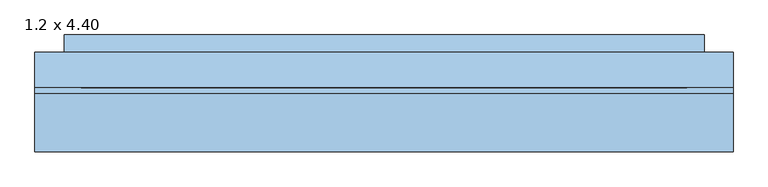
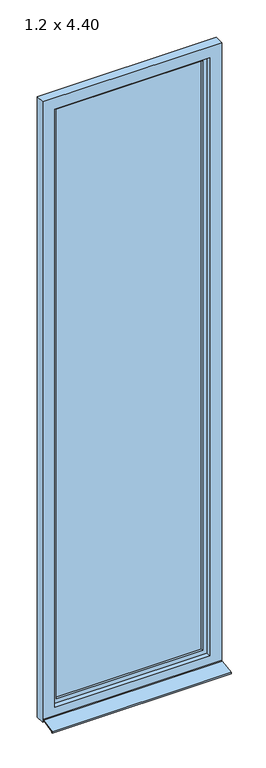
"""IFC4 building model written with IfcOpenShell, lengths in millimetres: window geometry, Fenstertür 1-flg : 1.2 x 4.40."""

from ifc_helpers import new_model, si_unit, frame, origin, place, context, project, spatial, polyline, outline, extrude, faceted_brep, source, transform, mapped, element, save


def window_1_2_x_4_40_89d25765(model_context):
    return source(origin(), model_context, "Body", "SolidModel", [
        extrude(outline(polyline([(4400.0, 600.0), (4400.0, -600.0), (0.0, -600.0), (0.0, 600.0), (4400.0, 600.0)]), holes=[polyline([(4320.0, 520.0), (80.0, 520.0), (80.0, -520.0), (4320.0, -520.0), (4320.0, 520.0)])]), frame((0.0, -70.0, 0.0), z_axis=(0.0, 1.0, 0.0), x_axis=(0.0, 0.0, 1.0)), (0.0, 0.0, 1.0), 60.0),
        faceted_brep([(550.0, -10.0, 4350.0), (550.0, -10.0, 50.0), (550.0, 20.0, 50.0), (550.0, 20.0, 4350.0), (-550.0, 20.0, 50.0), (-550.0, 20.0, 4350.0), (490.0, 20.0, 110.0), (490.0, 20.0, 4290.0), (-490.0, 20.0, 4290.0), (-490.0, 20.0, 110.0), (-550.0, -10.0, 50.0), (-550.0, -10.0, 4350.0), (520.0, -10.0, 4320.0), (520.0, -10.0, 80.0), (-520.0, -10.0, 80.0), (-520.0, -10.0, 4320.0), (520.0, -40.0, 4320.0), (520.0, -40.0, 80.0), (-520.0, -40.0, 80.0), (-520.0, -40.0, 4320.0), (490.0, -40.0, 4290.0), (490.0, -40.0, 110.0), (-490.0, -40.0, 110.0), (-490.0, -40.0, 4290.0)], [[[0, 1, 2, 3]], [[3, 2, 4, 5], [6, 7, 8, 9]], [[1, 10, 4, 2]], [[1, 0, 11, 10], [12, 13, 14, 15]], [[16, 17, 13, 12]], [[17, 18, 14, 13]], [[17, 16, 19, 18], [20, 21, 22, 23]], [[7, 6, 21, 20]], [[6, 9, 22, 21]], [[10, 11, 5, 4]], [[18, 19, 15, 14]], [[9, 8, 23, 22]], [[11, 0, 3, 5]], [[19, 16, 12, 15]], [[8, 7, 20, 23]]]),
        extrude(outline(polyline([(-80.0221543, 20.0), (-70.0, 20.0), (-70.0, 18.0), (-79.8240723, 18.0), (-178.0, -1.6395366), (-178.0, -10.0), (-180.0, -10.0), (-180.0, 0.0), (-80.0221543, 20.0)])), frame((-600.0, 0.0, 0.0), z_axis=(1.0, 0.0, 0.0), x_axis=(0.0, 1.0, 0.0)), (0.0, 0.0, 1.0), 1200.0),
        extrude(outline(polyline([(490.0, 5.0), (490.0, -25.0), (-490.0, -25.0), (-490.0, 5.0), (490.0, 5.0)])), frame((0.0, 0.0, 110.0), z_axis=(0.0, 0.0, 1.0), x_axis=(1.0, 0.0, 0.0)), (0.0, 0.0, 1.0), 4180.0),
    ])


if __name__ == "__main__":
    model = new_model("IFC4")
    model_context = context("Model", 3, world=origin())
    ifc_project = project(units=[si_unit("LENGTHUNIT", "METRE", prefix="MILLI")], contexts=[model_context])
    site = spatial("IfcSite", under=ifc_project)
    building = spatial("IfcBuilding", under=site)
    placement = place(None, origin())
    window_1_2_x_4_40_shape = window_1_2_x_4_40_89d25765(model_context)
    element("IfcWindow", 1, ObjectType="Fenstertür 1-flg : 1.2 x 4.40", at=placement, inside=building, context=model_context, shape_type="MappedRepresentation", body=[
        mapped(window_1_2_x_4_40_shape, transform((0.0, 0.0, 0.0), x_axis=(1.0, 0.0, 0.0), y_axis=(0.0, 1.0, 0.0), z_axis=(0.0, 0.0, 1.0))),
    ])
    save(model, "model.ifc")

# Revit data of these elements
# Type "Fenstertür 1-flg : 1.2 x 4.40"
#   Type Mark = "56"
#   Operation = "SinglePanel"
#   Construction Type Id = "GSP4R"
#   Keynote = "16.05.01"
#   Analytic Construction = "1/8 Zoll Pilkington-Verglasung einfach"
#   Visual Light Transmittance = 0.9
#   Thermal Resistance (R) = 0.1491 (m²·K)/W
#   Solar Heat Gain Coefficient = 0.86
#   Rough Width = 1.200 m
#   Rough Height = 4.400 m
#   Heat Transfer Coefficient (U) = 6.7069 W/(m²·K)
#   Rahmentiefe = 0.060 m
#   Rahmenhöhe - unten = 0.080 m
#   Rahmenhöhe - oben = 0.080 m
#   Rahmenbreite = 0.080 m
#   Height = 4.400 m
#   Tiefe Flügel = 0.060 m
#   Flügelbreite = 0.060 m
#   Einbautiefe (von außen) [instance default] = 0.080 m
#   Width = 1.200 m
#   Kippflügel [instance default] = yes
#   Drehflügel im Grundriss darstellen [instance default] = yes
#   Drehflügel 1 [instance default] = yes
#   Rahmen 1 [instance default] = none
#   Glas [instance default] = none
#   Flügel [instance default] = none
#   Fensterbank Außenseite [instance default] = none
#   Wall Closure = (empty or 0)
# Element 1 (IfcWindow, "Fenstertür 1-flg : 1.2 x 4.40")
#   Materials on its faces: "Kunststoff - Weiß", "Glas"
# Materials
#   "Kunststoff - Weiß": class "Kunststoff", colour RGB 249 249 249, transparency 0, Cost = 0
#   "Glas": class "Glas", colour RGB 0 0 255, transparency 0.75, Comments = "Render-Darstellung nicht aktualisiert ", Cost = 0
